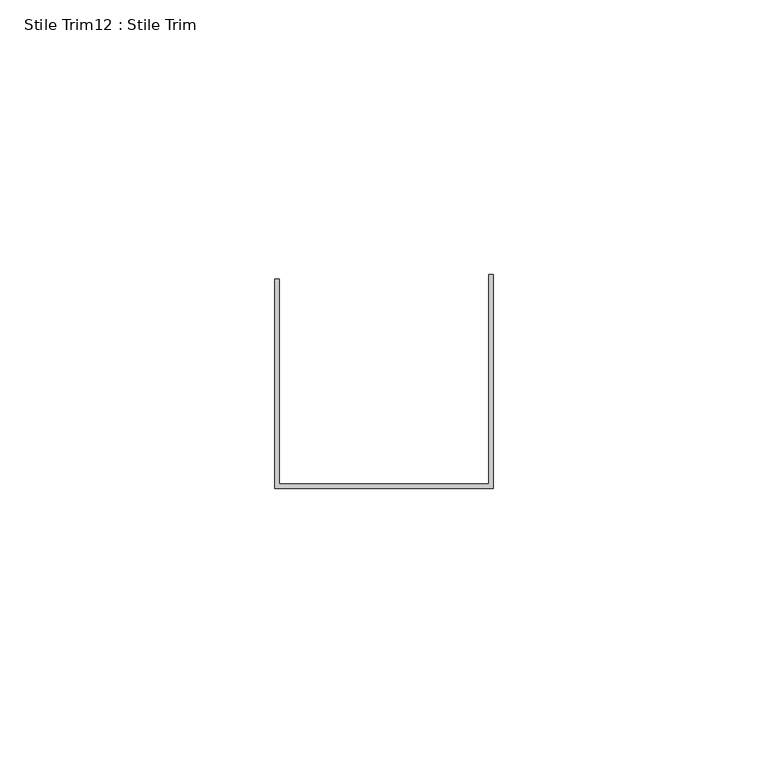
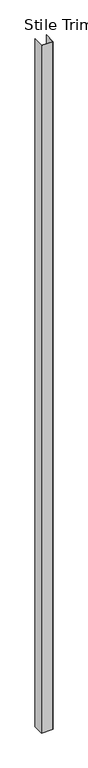
"""IFC4 building model written with IfcOpenShell, lengths in millimetres: proxy geometry, Stile Trim12 : Stile Trim."""

from ifc_helpers import new_model, si_unit, origin, origin_with_axes, place, context, project, spatial, polyline, outline, extrude, source, transform, mapped, element, save


def stile_trim12_stile_trim_a5a4c22f(model_context):
    return source(origin(), model_context, "Body", "SweptSolid", [
        extrude(outline(polyline([(590392.4558739, -536420.7663841), (590352.7810739, -536420.7663841), (590352.7810739, -536382.6663841), (590353.5684739, -536382.6663841), (590353.5684739, -536419.9789841), (590391.6684739, -536419.9789841), (590391.6684739, -536381.8789841), (590392.4558739, -536381.8789841), (590392.4558739, -536420.7663841)])), origin_with_axes(), (0.0, 0.0, 1.0), 2438.4),
    ])


if __name__ == "__main__":
    model = new_model("IFC4")
    model_context = context("Model", 3, world=origin())
    ifc_project = project(units=[si_unit("LENGTHUNIT", "METRE", prefix="MILLI")], contexts=[model_context])
    site = spatial("IfcSite", under=ifc_project)
    building = spatial("IfcBuilding", under=site)
    placement = place(None, origin())
    stile_trim12_stile_trim_shape = stile_trim12_stile_trim_a5a4c22f(model_context)
    element("IfcBuildingElementProxy", 1, Name="Stile Trim12 : Stile Trim", ObjectType="Stile Trim12 : Stile Trim", at=placement, inside=building, context=model_context, shape_type="MappedRepresentation", body=[
        mapped(stile_trim12_stile_trim_shape, transform((0.0, 0.0, 0.0), x_axis=(1.0, 0.0, 0.0), y_axis=(0.0, 1.0, 0.0), z_axis=(0.0, 0.0, 1.0))),
    ])
    save(model, "model.ifc")

# Revit data of these elements
# Element 1 (IfcBuildingElementProxy, "Stile Trim12 : Stile Trim")
#   Materials on its faces: "EDGE TRIM BY MTL PANEL MFR."
# Materials
#   "EDGE TRIM BY MTL PANEL MFR.": class "Generic", colour RGB 239 242 240, transparency 0, Cost = 0
